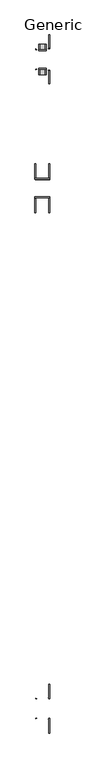
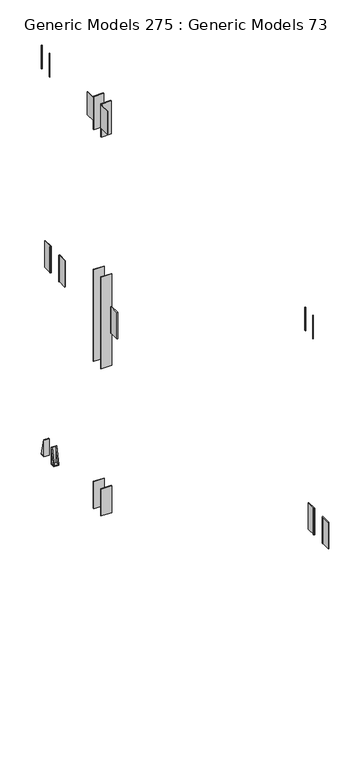
"""IFC4 building model written with IfcOpenShell, lengths in millimetres: proxy geometry, Generic Models 275 : Generic Models 73."""

from ifc_helpers import new_model, si_unit, frame, origin, place, context, project, spatial, polyline, outline, extrude, source, transform, mapped, element, save


def generic_models_275_generic_models_73_4b9bd806(model_context):
    return source(origin(), model_context, "Body", "SweptSolid", [
        extrude(outline(polyline([(32045.2835525, 35213.6207942), (32053.2210525, 35213.6207942), (32053.2210525, 35078.6832942), (32045.2835525, 35078.6832942), (32045.2835525, 35213.6207942)])), frame((0.0, 0.0, 268776.45), z_axis=(0.0, 0.0, 1.0), x_axis=(1.0, 0.0, 0.0)), (0.0, 0.0, 1.0), 342.9),
        extrude(outline(polyline([(32053.2090778, 35213.6207942), (32053.2090778, 35205.6832942), (31926.2090778, 35205.6832942), (31926.2090778, 35213.6207942), (32053.2090778, 35213.6207942)])), frame((0.0, 0.0, 266430.125), z_axis=(0.0, 0.0, 1.0), x_axis=(1.0, 0.0, 0.0)), (0.0, 0.0, 1.0), 348.4501684),
        extrude(outline(polyline([(32053.2090778, 35373.9582942), (32053.2090778, 35366.0207942), (31926.2090778, 35366.0207942), (31926.2090778, 35373.9582942), (32053.2090778, 35373.9582942)])), frame((0.0, 0.0, 266430.125), z_axis=(0.0, 0.0, 1.0), x_axis=(1.0, 0.0, 0.0)), (0.0, 0.0, 1.0), 348.4501684),
        extrude(outline(polyline([(32053.2090778, 35373.9582942), (32053.2090778, 35366.0207942), (31926.2090778, 35366.0207942), (31926.2090778, 35373.9582942), (32053.2090778, 35373.9582942)])), frame((0.0, 0.0, 268349.4125), z_axis=(0.0, 0.0, 1.0), x_axis=(1.0, 0.0, 0.0)), (0.0, 0.0, 1.0), 1195.3875),
        extrude(outline(polyline([(32053.2090778, 35213.6207942), (32053.2090778, 35205.6832942), (31926.2090778, 35205.6832942), (31926.2090778, 35213.6207942), (32053.2090778, 35213.6207942)])), frame((0.0, 0.0, 268349.4125), z_axis=(0.0, 0.0, 1.0), x_axis=(1.0, 0.0, 0.0)), (0.0, 0.0, 1.0), 1195.3875),
        extrude(outline(polyline([(36540.7707942, 266422.1875), (36491.5582942, 266422.1875), (36491.5582942, 266633.325), (36540.7707942, 266422.1875)])), frame((32011.9340778, 0.0, 0.0), z_axis=(1.0, 0.0, 0.0), x_axis=(0.0, 1.0, 0.0)), (0.0, 0.0, 1.0), 7.9375),
        extrude(outline(polyline([(36274.0707942, 266422.1875), (36323.2832942, 266633.325), (36323.2832942, 266422.1875), (36274.0707942, 266422.1875)])), frame((32011.9340778, 0.0, 0.0), z_axis=(1.0, 0.0, 0.0), x_axis=(0.0, 1.0, 0.0)), (0.0, 0.0, 1.0), 7.9375),
        extrude(outline(polyline([(32045.2835525, 30688.6156612), (32053.2210525, 30688.6156612), (32053.2210525, 30561.6156612), (32045.2835525, 30561.6156612), (32045.2835525, 30688.6156612)])), frame((0.0, 0.0, 268776.45), z_axis=(0.0, 0.0, 1.0), x_axis=(1.0, 0.0, 0.0)), (0.0, 0.0, 1.0), 342.9),
        extrude(outline(polyline([(32045.2835525, 30987.0656612), (32053.2210525, 30987.0656612), (32053.2210525, 30860.0656612), (32045.2835525, 30860.0656612), (32045.2835525, 30987.0656612)])), frame((0.0, 0.0, 268776.45), z_axis=(0.0, 0.0, 1.0), x_axis=(1.0, 0.0, 0.0)), (0.0, 0.0, 1.0), 342.9),
        extrude(outline(polyline([(31937.3215778, 35373.9582942), (31930.9715778, 35373.9582942), (31930.9715778, 35380.3082942), (31937.3215778, 35373.9582942)])), frame((0.0, 0.0, 271481.55), z_axis=(0.0, 0.0, 1.0), x_axis=(1.0, 0.0, 0.0)), (0.0, 0.0, 1.0), 304.8),
        extrude(outline(polyline([(31937.3215778, 35205.6832942), (31930.9715778, 35199.3332942), (31930.9715778, 35205.6832942), (31937.3215778, 35205.6832942)])), frame((0.0, 0.0, 271481.55), z_axis=(0.0, 0.0, 1.0), x_axis=(1.0, 0.0, 0.0)), (0.0, 0.0, 1.0), 304.8),
        extrude(outline(polyline([(31937.3215778, 36491.5582942), (31930.9715778, 36491.5582942), (31930.9715778, 36497.9082942), (31937.3215778, 36491.5582942)])), frame((0.0, 0.0, 271481.55), z_axis=(0.0, 0.0, 1.0), x_axis=(1.0, 0.0, 0.0)), (0.0, 0.0, 1.0), 304.8),
        extrude(outline(polyline([(31937.3215778, 36323.2832942), (31930.9715778, 36316.9332942), (31930.9715778, 36323.2832942), (31937.3215778, 36323.2832942)])), frame((0.0, 0.0, 271481.55), z_axis=(0.0, 0.0, 1.0), x_axis=(1.0, 0.0, 0.0)), (0.0, 0.0, 1.0), 304.8),
        extrude(outline(polyline([(31937.3215778, 30858.4781612), (31930.9715778, 30858.4781612), (31930.9715778, 30864.8281612), (31937.3215778, 30858.4781612)])), frame((0.0, 0.0, 271481.55), z_axis=(0.0, 0.0, 1.0), x_axis=(1.0, 0.0, 0.0)), (0.0, 0.0, 1.0), 304.8),
        extrude(outline(polyline([(31937.3215778, 30690.2031612), (31930.9715778, 30683.8531612), (31930.9715778, 30690.2031612), (31937.3215778, 30690.2031612)])), frame((0.0, 0.0, 271481.55), z_axis=(0.0, 0.0, 1.0), x_axis=(1.0, 0.0, 0.0)), (0.0, 0.0, 1.0), 304.8),
        extrude(outline(polyline([(36540.7707942, 266422.1875), (36491.5582942, 266422.1875), (36491.5582942, 266633.325), (36540.7707942, 266422.1875)])), frame((31956.3715778, 0.0, 0.0), z_axis=(1.0, 0.0, 0.0), x_axis=(0.0, 1.0, 0.0)), (0.0, 0.0, 1.0), 7.9375),
        extrude(outline(polyline([(36274.0707942, 266422.1875), (36323.2832942, 266633.325), (36323.2832942, 266422.1875), (36274.0707942, 266422.1875)])), frame((31956.3715778, 0.0, 0.0), z_axis=(1.0, 0.0, 0.0), x_axis=(0.0, 1.0, 0.0)), (0.0, 0.0, 1.0), 7.9375),
        extrude(outline(polyline([(36323.2832942, 266633.325), (36331.2207942, 266633.325), (36331.2207942, 266414.25), (36274.0707942, 266414.25), (36274.0707942, 266422.1875), (36323.2832942, 266422.1875), (36323.2832942, 266633.325)])), frame((31956.3715778, 0.0, 0.0), z_axis=(1.0, 0.0, 0.0), x_axis=(0.0, 1.0, 0.0)), (0.0, 0.0, 1.0), 63.5),
        extrude(outline(polyline([(36483.6207942, 266633.325), (36491.5582942, 266633.325), (36491.5582942, 266422.1875), (36540.7707942, 266422.1875), (36540.7707942, 266414.25), (36483.6207942, 266414.25), (36483.6207942, 266633.325)])), frame((31956.3715778, 0.0, 0.0), z_axis=(1.0, 0.0, 0.0), x_axis=(0.0, 1.0, 0.0)), (0.0, 0.0, 1.0), 63.5),
        extrude(outline(polyline([(32038.9215778, 35373.9582942), (32045.2715778, 35380.3082942), (32045.2715778, 35373.9582942), (32038.9215778, 35373.9582942)])), frame((0.0, 0.0, 268776.45), z_axis=(0.0, 0.0, 1.0), x_axis=(1.0, 0.0, 0.0)), (0.0, 0.0, 1.0), 342.9),
        extrude(outline(polyline([(32038.9215778, 35205.6832942), (32045.2715778, 35205.6832942), (32045.2715778, 35199.3332942), (32038.9215778, 35205.6832942)])), frame((0.0, 0.0, 268776.45), z_axis=(0.0, 0.0, 1.0), x_axis=(1.0, 0.0, 0.0)), (0.0, 0.0, 1.0), 342.9),
        extrude(outline(polyline([(32038.9215778, 36501.0832942), (32045.2715778, 36507.4332942), (32045.2715778, 36501.0832942), (32038.9215778, 36501.0832942)])), frame((0.0, 0.0, 268776.45), z_axis=(0.0, 0.0, 1.0), x_axis=(1.0, 0.0, 0.0)), (0.0, 0.0, 1.0), 342.9),
        extrude(outline(polyline([(32038.9215778, 36313.7582942), (32045.2715778, 36313.7582942), (32045.2715778, 36307.4082942), (32038.9215778, 36313.7582942)])), frame((0.0, 0.0, 268776.45), z_axis=(0.0, 0.0, 1.0), x_axis=(1.0, 0.0, 0.0)), (0.0, 0.0, 1.0), 342.9),
        extrude(outline(polyline([(32038.9215778, 30868.0031612), (32045.2715778, 30874.3531612), (32045.2715778, 30868.0031612), (32038.9215778, 30868.0031612)])), frame((0.0, 0.0, 268776.45), z_axis=(0.0, 0.0, 1.0), x_axis=(1.0, 0.0, 0.0)), (0.0, 0.0, 1.0), 342.9),
        extrude(outline(polyline([(32038.9215778, 30680.6781612), (32045.2715778, 30680.6781612), (32045.2715778, 30674.3281612), (32038.9215778, 30680.6781612)])), frame((0.0, 0.0, 268776.45), z_axis=(0.0, 0.0, 1.0), x_axis=(1.0, 0.0, 0.0)), (0.0, 0.0, 1.0), 342.9),
        extrude(outline(polyline([(32045.2835525, 36313.7582942), (32053.2210525, 36313.7582942), (32053.2210525, 36194.6957942), (32045.2835525, 36194.6957942), (32045.2835525, 36313.7582942)])), frame((0.0, 0.0, 268776.45), z_axis=(0.0, 0.0, 1.0), x_axis=(1.0, 0.0, 0.0)), (0.0, 0.0, 1.0), 342.9),
        extrude(outline(polyline([(32045.2835525, 36620.1457942), (32053.2210525, 36620.1457942), (32053.2210525, 36501.0832942), (32045.2835525, 36501.0832942), (32045.2835525, 36620.1457942)])), frame((0.0, 0.0, 268776.45), z_axis=(0.0, 0.0, 1.0), x_axis=(1.0, 0.0, 0.0)), (0.0, 0.0, 1.0), 342.9),
        extrude(outline(polyline([(31923.0340778, 35213.6207942), (31930.9715778, 35213.6207942), (31930.9715778, 35078.6832942), (31923.0340778, 35078.6832942), (31923.0340778, 35213.6207942)])), frame((0.0, 0.0, 271490.7765953), z_axis=(0.0, 0.0, 1.0), x_axis=(1.0, 0.0, 0.0)), (0.0, 0.0, 1.0), 295.5734047),
        extrude(outline(polyline([(31923.0340778, 35500.9582942), (31930.9715778, 35500.9582942), (31930.9715778, 35373.9582942), (31923.0340778, 35373.9582942), (31923.0340778, 35500.9582942)])), frame((0.0, 0.0, 271490.7765953), z_axis=(0.0, 0.0, 1.0), x_axis=(1.0, 0.0, 0.0)), (0.0, 0.0, 1.0), 295.5734047),
        extrude(outline(polyline([(32045.2835525, 35500.9582942), (32053.2210525, 35500.9582942), (32053.2210525, 35366.0207942), (32045.2835525, 35366.0207942), (32045.2835525, 35500.9582942)])), frame((0.0, 0.0, 268776.45), z_axis=(0.0, 0.0, 1.0), x_axis=(1.0, 0.0, 0.0)), (0.0, 0.0, 1.0), 342.9),
        extrude(outline(polyline([(32050.0340778, 35213.6207942), (32050.0340778, 35205.6832942), (31923.0340778, 35205.6832942), (31923.0340778, 35213.6207942), (32050.0340778, 35213.6207942)])), frame((0.0, 0.0, 271373.8984047), z_axis=(0.0, 0.0, 1.0), x_axis=(1.0, 0.0, 0.0)), (0.0, 0.0, 1.0), 431.5015953),
        extrude(outline(polyline([(32050.0340778, 35373.9582942), (32050.0340778, 35366.0207942), (31923.0340778, 35366.0207942), (31923.0340778, 35373.9582942), (32050.0340778, 35373.9582942)])), frame((0.0, 0.0, 271373.8984047), z_axis=(0.0, 0.0, 1.0), x_axis=(1.0, 0.0, 0.0)), (0.0, 0.0, 1.0), 431.5015953),
    ])


if __name__ == "__main__":
    model = new_model("IFC4")
    model_context = context("Model", 3, world=origin())
    ifc_project = project(units=[si_unit("LENGTHUNIT", "METRE", prefix="MILLI")], contexts=[model_context])
    site = spatial("IfcSite", under=ifc_project)
    building = spatial("IfcBuilding", under=site)
    placement = place(None, origin())
    generic_models_275_generic_models_73_shape = generic_models_275_generic_models_73_4b9bd806(model_context)
    element("IfcBuildingElementProxy", 1, Name="Generic Models 275 : Generic Models 73", ObjectType="Generic Models 275 : Generic Models 73", at=placement, inside=building, context=model_context, shape_type="MappedRepresentation", body=[
        mapped(generic_models_275_generic_models_73_shape, transform((0.0, 0.0, 0.0), x_axis=(1.0, 0.0, 0.0), y_axis=(0.0, 1.0, 0.0), z_axis=(0.0, 0.0, 1.0))),
    ])
    save(model, "model.ifc")

# Revit data of these elements
# Element 1 (IfcBuildingElementProxy, "Generic Models 275 : Generic Models 73")
#   Materials on its faces: "5/16\" THICK GALV. STEEL PLATE", "FULL LENGTH WELD", "SIMPSON HD3B GALV. HOLDDOWN", "5/16 x 5\" WIDE SIDE PLATES 3/4\"DIA. THRU BOLTS"
# Materials
#   "5/16\" THICK GALV. STEEL PLATE": class "Metal", colour RGB 199 199 199, transparency 0, Description = "Carbon steel", Cost = 0
#   "FULL LENGTH WELD": class "Metal", colour RGB 199 199 199, transparency 0, Description = "Carbon steel", Cost = 0
#   "SIMPSON HD3B GALV. HOLDDOWN": class "Metal", colour RGB 199 199 199, transparency 0, Description = "Carbon steel", Cost = 0
#   "5/16 x 5\" WIDE SIDE PLATES 3/4\"DIA. THRU BOLTS": class "Metal", colour RGB 199 199 199, transparency 0, Description = "Carbon steel", Cost = 0
